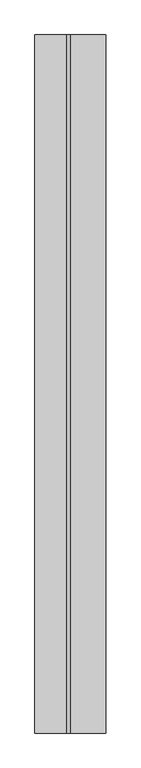
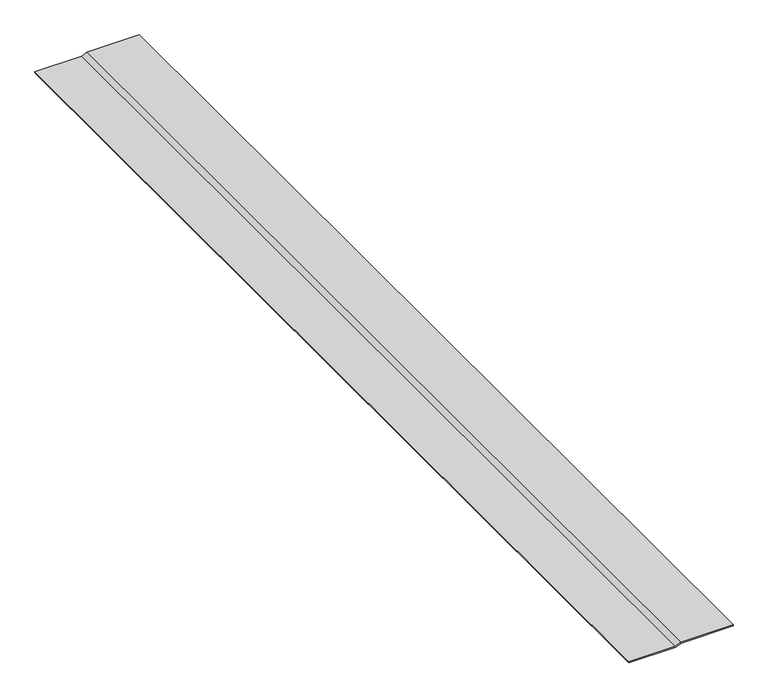
"""IFC4 building model written with IfcOpenShell, lengths in millimetres: proxy geometry, INTERPLY002 : INTERPLY002."""

from ifc_helpers import new_model, si_unit, frame, origin, place, context, project, spatial, polyline, outline, extrude, source, transform, mapped, element, save


def generic_models_8be46f14(model_context):
    return source(origin(), model_context, "Body", "SweptSolid", [
        extrude(outline(polyline([(40265.8733085, -4491.2259186), (40261.1620854, -4501.7914992), (40261.1620854, -4592.5295682), (40258.8529944, -4592.5295682), (40258.8529944, -4501.3000079), (40263.5642176, -4490.7344272), (40263.5642176, -4389.4895292), (40265.8733085, -4389.4895292), (40265.8733085, -4491.2259186)])), frame((0.0, -1065.5906573, 0.0), z_axis=(0.0, 1.0, 0.0), x_axis=(0.0, 0.0, 1.0)), (0.0, 0.0, 1.0), 2000.25),
    ])


if __name__ == "__main__":
    model = new_model("IFC4")
    model_context = context("Model", 3, world=origin())
    ifc_project = project(units=[si_unit("LENGTHUNIT", "METRE", prefix="MILLI")], contexts=[model_context])
    site = spatial("IfcSite", under=ifc_project)
    building = spatial("IfcBuilding", under=site)
    placement = place(None, origin())
    generic_models_shape = generic_models_8be46f14(model_context)
    element("IfcBuildingElementProxy", 1, Name="INTERPLY002 : INTERPLY002", ObjectType="INTERPLY002 : INTERPLY002", at=placement, inside=building, context=model_context, shape_type="MappedRepresentation", body=[
        mapped(generic_models_shape, transform((0.0, 0.0, 0.0), x_axis=(1.0, 0.0, 0.0), y_axis=(0.0, 1.0, 0.0), z_axis=(0.0, 0.0, 1.0))),
    ])
    save(model, "model.ifc")

# Revit data of these elements
# Type "INTERPLY002 : INTERPLY002"
#   NameOverride = "INTERPLY002"
# Element 1 (IfcBuildingElementProxy, "INTERPLY002 : INTERPLY002")
#   Materials on its faces: "INTERPLY REQUIRED FOR 15 & 20 YEARS SYSTEMS"
# Materials
#   "INTERPLY REQUIRED FOR 15 & 20 YEARS SYSTEMS": class "Unassigned", colour RGB 115 115 172, transparency 0
